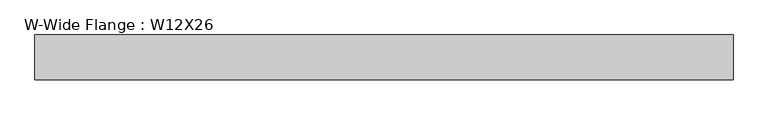
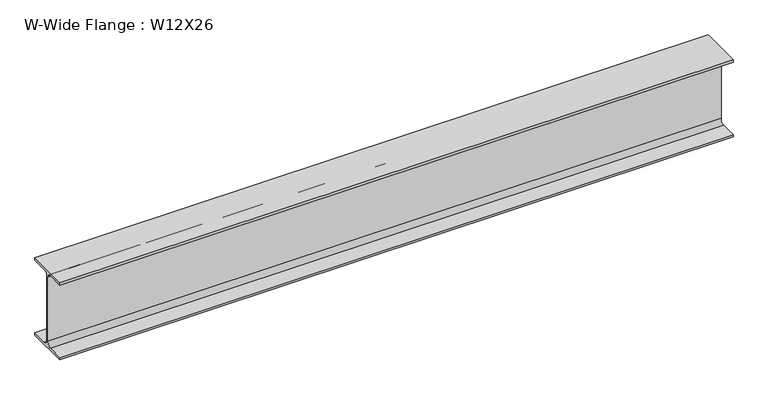
"""IFC4 building model written with IfcOpenShell, lengths in millimetres: beam geometry, W-Wide Flange : W12X26."""

from ifc_helpers import new_model, si_unit, point, frame, frame_2d, origin, place, context, project, spatial, polyline, circle_curve, trimmed, segment, composite_curve, outline, extrude, source, transform, mapped, element, save


def w_wide_flange_w12x26_a858fbf7(model_context):
    return source(origin(), model_context, "Body", "SweptSolid", [
        extrude(outline(composite_curve([segment(polyline([(-82.4011719, -145.5539063), (-20.2902344, -145.5539063)]), True, "CONTINUOUS"), segment(trimmed(circle_curve(frame_2d((-20.2902344, -128.190625)), 17.3632812), [point((-20.2902344, -145.5539063))], [point((-2.9269531, -128.190625))], True, "CARTESIAN"), True, "CONTINUOUS"), segment(polyline([(-2.9269531, -128.190625), (-2.9269531, 128.190625)]), True, "CONTINUOUS"), segment(trimmed(circle_curve(frame_2d((-20.2902344, 128.190625)), 17.3632812), [point((-2.9269531, 128.190625))], [point((-20.2902344, 145.5539062))], True, "CARTESIAN"), True, "CONTINUOUS"), segment(polyline([(-20.2902344, 145.5539062), (-82.4011719, 145.5539062), (-82.4011719, 155.178125), (82.4011719, 155.178125), (82.4011719, 145.5539062), (20.2902344, 145.5539062)]), True, "CONTINUOUS"), segment(trimmed(circle_curve(frame_2d((20.2902344, 128.190625)), 17.3632812), [point((20.2902344, 145.5539062))], [point((2.9269531, 128.190625))], True, "CARTESIAN"), True, "CONTINUOUS"), segment(polyline([(2.9269531, 128.190625), (2.9269531, -128.190625)]), True, "CONTINUOUS"), segment(trimmed(circle_curve(frame_2d((20.2902344, -128.190625)), 17.3632812), [point((2.9269531, -128.190625))], [point((20.2902344, -145.5539063))], True, "CARTESIAN"), True, "CONTINUOUS"), segment(polyline([(20.2902344, -145.5539063), (82.4011719, -145.5539063), (82.4011719, -155.178125), (-82.4011719, -155.178125), (-82.4011719, -145.5539063)]), True, "CONTINUOUS")], self_intersect=False)), frame((-1282.7, 0.0, 0.0), z_axis=(1.0, 0.0, 0.0), x_axis=(0.0, 1.0, 0.0)), (0.0, 0.0, 1.0), 2559.05),
    ])


if __name__ == "__main__":
    model = new_model("IFC4")
    model_context = context("Model", 3, world=origin())
    ifc_project = project(units=[si_unit("LENGTHUNIT", "METRE", prefix="MILLI")], contexts=[model_context])
    site = spatial("IfcSite", under=ifc_project)
    building = spatial("IfcBuilding", under=site)
    placement = place(None, origin())
    w_wide_flange_w12x26_shape = w_wide_flange_w12x26_a858fbf7(model_context)
    element("IfcBeam", 1, ObjectType="W-Wide Flange : W12X26", at=placement, inside=building, context=model_context, shape_type="MappedRepresentation", body=[
        mapped(w_wide_flange_w12x26_shape, transform((0.0, 0.0, 0.0), x_axis=(1.0, 0.0, 0.0), y_axis=(0.0, 1.0, 0.0), z_axis=(0.0, 0.0, 1.0))),
    ])
    save(model, "model.ifc")

# Revit data of these elements
# Type "W-Wide Flange : W12X26"
#   Assembly Code = "B10"
#   W = 26
#   Start Extension Calculation [instance default] = 10' - 0"
#   Start Extension [instance default] = -0' - 0 1/2"
#   End Extension Calculation [instance default] = 10' - 0"
#   End Extension [instance default] = -0' - 0 1/2"
#   Length [instance default] = 5' - 0"
#   bf = 0' - 6 125/256"
#   d = 1' - 0 7/32"
#   k = 0' - 1 1/16"
#   k2 = 0' - 0 175/256"
#   tf = 0' - 0 97/256"
#   tw = 0' - 0 59/256"
#   A = 0.05 SF
#   Beam Material [instance default] = Metal - Steel - ASTM A992
# Element 1 (IfcBeam, "W-Wide Flange : W12X26")
#   Materials on its faces: "Metal - Steel - ASTM A992"
# Materials
#   "Metal - Steel - ASTM A992": class "Metal", colour RGB 128 0 0, transparency 0
